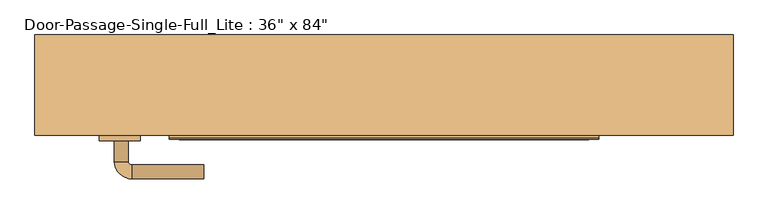
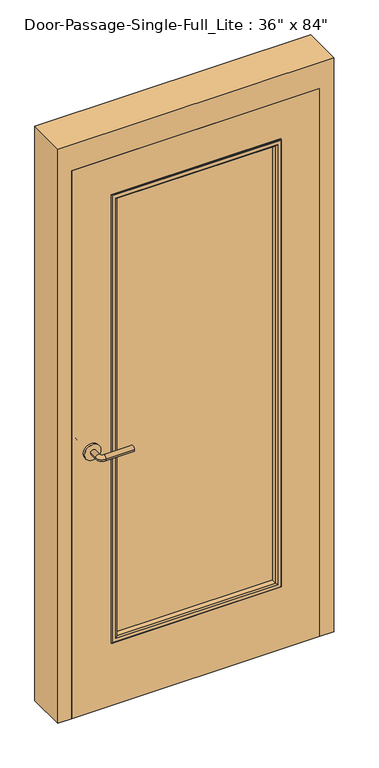
"""IFC4 building model written with IfcOpenShell, lengths in millimetres: door geometry."""

from ifc_helpers import new_model, si_unit, point, frame, frame_2d, origin, place, context, project, spatial, polyline, circle_curve, ellipse_curve, trimmed, segment, composite_curve, outline, extrude, faceted_brep, source, transform, mapped, element, save
from ifc_brep_helpers import plane_surface, cylinder_surface, revolved_surface, advanced_brep


def door_4cfbdd5f(model_context):
    return source(origin(), model_context, "Body", "SolidModel", [
        advanced_brep(
        [(-392.190625, -23.75, 1016.0), (-372.190625, -23.75, 1016.0), (-392.190625, 6.25, 1016.0), (-372.190625, 6.25, 1016.0), (-367.190625, 11.25, 1016.0), (-367.190625, 31.25, 1016.0), (-262.190625, 31.25, 1016.0), (-262.190625, 11.25, 1016.0)],
        [
            (0, 1, circle_curve(frame((-382.190625, -23.75, 1016.0), z_axis=(0.0, -1.0, 0.0), x_axis=(1.0, 0.0, 0.0)), 10.0)),
            (1, 0, circle_curve(frame((-382.190625, -23.75, 1016.0), z_axis=(0.0, -1.0, 0.0), x_axis=(1.0, 0.0, 0.0)), 10.0)),
            (0, 2),
            (2, 3, circle_curve(frame((-382.190625, 6.25, 1016.0), z_axis=(0.0, -1.0, 0.0), x_axis=(1.0, 0.0, 0.0)), 10.0)),
            (3, 1),
            (3, 2, circle_curve(frame((-382.190625, 6.25, 1016.0), z_axis=(0.0, -1.0, 0.0), x_axis=(1.0, 0.0, 0.0)), 10.0)),
            (4, 3, circle_curve(frame((-367.190625, 6.25, 1016.0), z_axis=(0.0, 0.0, 1.0), x_axis=(-1.0, 0.0, 0.0)), 5.0)),
            (2, 5, circle_curve(frame((-367.190625, 6.25, 1016.0), z_axis=(0.0, 0.0, -1.0), x_axis=(-1.0, 0.0, 0.0)), 25.0)),
            (5, 4, circle_curve(frame((-367.190625, 21.25, 1016.0), z_axis=(-1.0, 0.0, 0.0), x_axis=(0.0, -1.0, 0.0)), 10.0)),
            (4, 5, circle_curve(frame((-367.190625, 21.25, 1016.0), z_axis=(-1.0, 0.0, 0.0), x_axis=(0.0, -1.0, 0.0)), 10.0)),
            (6, 7, circle_curve(frame((-262.190625, 21.25, 1016.0), z_axis=(1.0, 0.0, 0.0), x_axis=(0.0, -1.0, 0.0)), 10.0)),
            (7, 6, circle_curve(frame((-262.190625, 21.25, 1016.0), z_axis=(1.0, 0.0, 0.0), x_axis=(0.0, -1.0, 0.0)), 10.0)),
            (5, 6),
            (7, 4),
        ],
        [
            plane_surface(frame((-382.190625, -23.75, 1016.0), z_axis=(0.0, -1.0, 0.0), x_axis=(0.0, 0.0, 1.0))),
            cylinder_surface(frame((-382.190625, -23.75, 1016.0), z_axis=(0.0, -1.0, 0.0), x_axis=(1.0, 0.0, 0.0)), 10.0),
            revolved_surface(trimmed(ellipse_curve(frame((-382.190625, 6.25, 1016.0), z_axis=(0.0, -1.0, 0.0), x_axis=(1.0, 0.0, 0.0)), 10.0, 10.0), [point((-392.190625, 6.25, 1016.0))], [point((-372.190625, 6.25, 1016.0))], True, "CARTESIAN"), (-367.190625, 6.25, 1016.0), (0.0, 0.0, -1.0)),
            revolved_surface(trimmed(ellipse_curve(frame((-382.190625, 6.25, 1016.0), z_axis=(0.0, -1.0, 0.0), x_axis=(1.0, 0.0, 0.0)), 10.0, 10.0), [point((-372.190625, 6.25, 1016.0))], [point((-392.190625, 6.25, 1016.0))], True, "CARTESIAN"), (-367.190625, 6.25, 1016.0), (0.0, 0.0, -1.0)),
            plane_surface(frame((-262.190625, 21.25, 1016.0), z_axis=(1.0, 0.0, 0.0), x_axis=(0.0, 0.0, 1.0))),
            cylinder_surface(frame((-367.190625, 21.25, 1016.0), z_axis=(-1.0, 0.0, 0.0), x_axis=(0.0, -1.0, 0.0)), 10.0),
        ],
        [
            (0, [[1, 2]]),
            (1, [[-1, 3, 4, 5]]),
            (1, [[-2, -5, 6, -3]]),
            (2, [[7, -4, 8, 9]]),
            (3, [[-8, -6, -7, 10]]),
            (4, [[11, 12]]),
            (5, [[-9, 13, -12, 14]]),
            (5, [[-10, -14, -11, -13]]),
        ],
    ),
        extrude(outline(composite_curve([segment(trimmed(circle_curve(frame_2d((1016.0, -384.690625)), 30.0), [point((1016.0, -414.690625))], [point((1016.0, -354.690625))], False, "CARTESIAN"), True, "CONTINUOUS"), segment(trimmed(circle_curve(frame_2d((1016.0, -384.690625)), 30.0), [point((1016.0, -354.690625))], [point((1016.0, -414.690625))], False, "CARTESIAN"), True, "CONTINUOUS")], self_intersect=False)), frame((0.0, -31.75, 0.0), z_axis=(0.0, 1.0, 0.0), x_axis=(0.0, 0.0, 1.0)), (0.0, 0.0, 1.0), 8.0),
        advanced_brep(
        [(-392.190625, -84.2, 1016.0), (-372.190625, -84.2, 1016.0), (-372.190625, -114.2, 1016.0), (-392.190625, -114.2, 1016.0), (-367.190625, -119.2, 1016.0), (-367.190625, -139.2, 1016.0), (-262.190625, -139.2, 1016.0), (-262.190625, -119.2, 1016.0)],
        [
            (0, 1, circle_curve(frame((-382.190625, -84.2, 1016.0), z_axis=(0.0, 1.0, 0.0), x_axis=(1.0, 0.0, 0.0)), 10.0)),
            (1, 0, circle_curve(frame((-382.190625, -84.2, 1016.0), z_axis=(0.0, 1.0, 0.0), x_axis=(1.0, 0.0, 0.0)), 10.0)),
            (1, 2),
            (2, 3, circle_curve(frame((-382.190625, -114.2, 1016.0), z_axis=(0.0, 1.0, 0.0), x_axis=(1.0, 0.0, 0.0)), 10.0)),
            (3, 0),
            (3, 2, circle_curve(frame((-382.190625, -114.2, 1016.0), z_axis=(0.0, 1.0, 0.0), x_axis=(1.0, 0.0, 0.0)), 10.0)),
            (4, 5, circle_curve(frame((-367.190625, -129.2, 1016.0), z_axis=(-1.0, 0.0, 0.0), x_axis=(0.0, 1.0, 0.0)), 10.0)),
            (5, 3, circle_curve(frame((-367.190625, -114.2, 1016.0), z_axis=(0.0, 0.0, -1.0), x_axis=(-1.0, 0.0, 0.0)), 25.0)),
            (2, 4, circle_curve(frame((-367.190625, -114.2, 1016.0), z_axis=(0.0, 0.0, 1.0), x_axis=(-1.0, 0.0, 0.0)), 5.0)),
            (5, 4, circle_curve(frame((-367.190625, -129.2, 1016.0), z_axis=(-1.0, 0.0, 0.0), x_axis=(0.0, 1.0, 0.0)), 10.0)),
            (6, 7, circle_curve(frame((-262.190625, -129.2, 1016.0), z_axis=(1.0, 0.0, 0.0), x_axis=(0.0, 1.0, 0.0)), 10.0)),
            (7, 6, circle_curve(frame((-262.190625, -129.2, 1016.0), z_axis=(1.0, 0.0, 0.0), x_axis=(0.0, 1.0, 0.0)), 10.0)),
            (4, 7),
            (6, 5),
        ],
        [
            plane_surface(frame((-382.190625, -84.2, 1016.0), z_axis=(0.0, 1.0, 0.0), x_axis=(0.0, 0.0, 1.0))),
            cylinder_surface(frame((-382.190625, -84.2, 1016.0), z_axis=(0.0, 1.0, 0.0), x_axis=(1.0, 0.0, 0.0)), 10.0),
            revolved_surface(trimmed(ellipse_curve(frame((-382.190625, -114.2, 1016.0), z_axis=(0.0, -1.0, 0.0), x_axis=(1.0, 0.0, 0.0)), 10.0, 10.0), [point((-392.190625, -114.2, 1016.0))], [point((-372.190625, -114.2, 1016.0))], True, "CARTESIAN"), (-367.190625, -114.2, 1016.0), (0.0, 0.0, -1.0)),
            revolved_surface(trimmed(ellipse_curve(frame((-382.190625, -114.2, 1016.0), z_axis=(0.0, -1.0, 0.0), x_axis=(1.0, 0.0, 0.0)), 10.0, 10.0), [point((-372.190625, -114.2, 1016.0))], [point((-392.190625, -114.2, 1016.0))], True, "CARTESIAN"), (-367.190625, -114.2, 1016.0), (0.0, 0.0, -1.0)),
            plane_surface(frame((-262.190625, -129.2, 1016.0), z_axis=(1.0, 0.0, 0.0), x_axis=(0.0, 0.0, 1.0))),
            cylinder_surface(frame((-367.190625, -129.2, 1016.0), z_axis=(-1.0, 0.0, 0.0), x_axis=(0.0, 1.0, 0.0)), 10.0),
        ],
        [
            (0, [[1, 2]]),
            (1, [[3, 4, 5, -2]]),
            (1, [[-5, 6, -3, -1]]),
            (2, [[7, 8, -4, 9]]),
            (3, [[10, -9, -6, -8]]),
            (4, [[11, 12]]),
            (5, [[13, -11, 14, -7]]),
            (5, [[-14, -12, -13, -10]]),
        ],
    ),
        extrude(outline(composite_curve([segment(trimmed(circle_curve(frame_2d((1016.0, -384.690625)), 30.0), [point((1016.0, -414.690625))], [point((1016.0, -354.690625))], False, "CARTESIAN"), True, "CONTINUOUS"), segment(trimmed(circle_curve(frame_2d((1016.0, -384.690625)), 30.0), [point((1016.0, -354.690625))], [point((1016.0, -414.690625))], False, "CARTESIAN"), True, "CONTINUOUS")], self_intersect=False)), frame((0.0, -84.2, 0.0), z_axis=(0.0, 1.0, 0.0), x_axis=(0.0, 0.0, 1.0)), (0.0, 0.0, 1.0), 8.0),
        extrude(outline(polyline([(304.8, -50.8), (304.8, -57.15), (-304.8, -57.15), (-304.8, -50.8), (304.8, -50.8)])), frame((0.0, 0.0, 254.0), z_axis=(0.0, 0.0, 1.0), x_axis=(1.0, 0.0, 0.0)), (0.0, 0.0, 1.0), 1727.2),
        faceted_brep([(457.2, -26.9875, 0.0), (441.325, -26.9875, 0.0), (441.325, 20.6375, 0.0), (457.2, 20.6375, 0.0), (457.2, 69.85, 0.0), (508.0, 69.85, 0.0), (508.0, -76.2, 0.0), (457.2, -76.2, 0.0), (457.2, -76.2, 2133.6), (457.2, -26.9875, 2133.6), (508.0, -76.2, 2235.2), (-508.0, -76.2, 2235.2), (-508.0, -76.2, 0.0), (-457.2, -76.2, 0.0), (-457.2, -76.2, 2133.6), (508.0, 69.85, 2235.2), (457.2, 69.85, 2133.6), (-457.2, 69.85, 2133.6), (-457.2, 69.85, 0.0), (-508.0, 69.85, 0.0), (-508.0, 69.85, 2235.2), (457.2, 20.6375, 2133.6), (441.325, 20.6375, 2117.725), (-441.325, 20.6375, 2117.725), (-441.325, 20.6375, 0.0), (-457.2, 20.6375, 0.0), (-457.2, 20.6375, 2133.6), (441.325, -26.9875, 2117.725), (-457.2, -26.9875, 2133.6), (-457.2, -26.9875, 0.0), (-441.325, -26.9875, 0.0), (-441.325, -26.9875, 2117.725)], [[[0, 1, 2, 3, 4, 5, 6, 7]], [[7, 8, 9, 0]], [[6, 10, 11, 12, 13, 14, 8, 7]], [[5, 15, 10, 6]], [[4, 16, 17, 18, 19, 20, 15, 5]], [[3, 21, 16, 4]], [[2, 22, 23, 24, 25, 26, 21, 3]], [[1, 27, 22, 2]], [[0, 9, 28, 29, 30, 31, 27, 1]], [[8, 14, 28, 9]], [[16, 21, 26, 17]], [[22, 27, 31, 23]], [[12, 19, 18, 25, 24, 30, 29, 13]], [[13, 29, 28, 14]], [[11, 20, 19, 12]], [[17, 26, 25, 18]], [[23, 31, 30, 24]], [[15, 20, 11, 10]]]),
        extrude(outline(polyline([(2133.6, -457.2), (0.0, -457.2), (0.0, 457.2), (2133.6, 457.2), (2133.6, -457.2)]), holes=[polyline([(1981.2, -304.8), (1981.2, 304.8), (254.0, 304.8), (254.0, -304.8), (1981.2, -304.8)])]), frame((0.0, -76.2, 0.0), z_axis=(0.0, 1.0, 0.0), x_axis=(0.0, 0.0, 1.0)), (0.0, 0.0, 1.0), 44.45),
        advanced_brep(
        [(-304.8, -57.15, 1981.2), (-304.8, -57.15, 254.0), (-304.8, -76.2, 254.0), (-304.8, -76.2, 1981.2), (-292.8, -77.2, 1969.2), (-292.8, -77.2, 266.0), (-292.8, -57.15, 266.0), (-292.8, -57.15, 1969.2), (-297.8, -82.2, 1974.2), (-297.8, -82.2, 261.0), (-312.8, -80.2, 1989.2), (-312.8, -80.2, 246.0), (-310.8, -82.2, 248.0), (-310.8, -82.2, 1987.2), (-312.8, -76.2, 1989.2), (-312.8, -76.2, 246.0), (304.8, -57.15, 254.0), (304.8, -76.2, 254.0), (292.8, -77.2, 266.0), (292.8, -57.15, 266.0), (297.8, -82.2, 261.0), (312.8, -80.2, 246.0), (310.8, -82.2, 248.0), (312.8, -76.2, 246.0), (304.8, -57.15, 1981.2), (304.8, -76.2, 1981.2), (292.8, -77.2, 1969.2), (292.8, -57.15, 1969.2), (297.8, -82.2, 1974.2), (312.8, -80.2, 1989.2), (310.8, -82.2, 1987.2), (312.8, -76.2, 1989.2)],
        [
            (0, 1),
            (1, 2),
            (2, 3),
            (3, 0),
            (4, 5),
            (5, 6),
            (6, 7),
            (7, 4),
            (8, 9),
            (9, 5, ellipse_curve(frame((-297.8, -77.2, 261.0), z_axis=(-0.7071067811865475, 0.0, 0.7071067811865475), x_axis=(0.7071067811865474, 0.0, 0.7071067811865476)), 7.0710678, 5.0)),
            (4, 8, ellipse_curve(frame((-297.8, -77.2, 1974.2), z_axis=(-0.7071067811865475, 0.0, -0.7071067811865475), x_axis=(-0.7071067811865474, 0.0, 0.7071067811865476)), 7.0710678, 5.0)),
            (10, 11),
            (11, 12, ellipse_curve(frame((-310.8, -80.2, 248.0), z_axis=(-0.7071067811865475, 0.0, 0.7071067811865475), x_axis=(0.7071067811865474, 0.0, 0.7071067811865476)), 2.8284271, 2.0)),
            (12, 13),
            (13, 10, ellipse_curve(frame((-310.8, -80.2, 1987.2), z_axis=(-0.7071067811865475, 0.0, -0.7071067811865475), x_axis=(-0.7071067811865474, 0.0, 0.7071067811865476)), 2.8284271, 2.0)),
            (14, 15),
            (15, 11),
            (10, 14),
            (1, 16),
            (16, 17),
            (17, 2),
            (5, 18),
            (18, 19),
            (19, 6),
            (9, 20),
            (20, 18, ellipse_curve(frame((297.8, -77.2, 261.0), z_axis=(-0.7071067811865475, 0.0, -0.7071067811865475), x_axis=(-0.7071067811865476, 0.0, 0.7071067811865474)), 7.0710678, 5.0)),
            (11, 21),
            (21, 22, ellipse_curve(frame((310.8, -80.2, 248.0), z_axis=(-0.7071067811865475, 0.0, -0.7071067811865475), x_axis=(-0.7071067811865476, 0.0, 0.7071067811865474)), 2.8284271, 2.0)),
            (22, 12),
            (15, 23),
            (23, 21),
            (16, 24),
            (24, 25),
            (25, 17),
            (18, 26),
            (26, 27),
            (27, 19),
            (20, 28),
            (28, 26, ellipse_curve(frame((297.8, -77.2, 1974.2), z_axis=(0.7071067811865475, 0.0, -0.7071067811865475), x_axis=(-0.7071067811865474, 0.0, -0.7071067811865476)), 7.0710678, 5.0)),
            (21, 29),
            (29, 30, ellipse_curve(frame((310.8, -80.2, 1987.2), z_axis=(0.7071067811865475, 0.0, -0.7071067811865475), x_axis=(-0.7071067811865474, 0.0, -0.7071067811865476)), 2.8284271, 2.0)),
            (30, 22),
            (23, 31),
            (31, 29),
            (14, 31),
            (25, 3),
            (24, 0),
            (27, 7),
            (26, 4),
            (28, 8),
            (30, 13),
            (29, 10),
        ],
        [
            plane_surface(frame((-304.8, -76.2, 1981.2), z_axis=(-1.0, 0.0, 0.0), x_axis=(0.0, 0.0, -1.0))),
            plane_surface(frame((-292.8, -57.15, 1969.2), z_axis=(1.0, 0.0, 0.0), x_axis=(0.0, 0.0, -1.0))),
            cylinder_surface(frame((-297.8, -77.2, 1981.2), z_axis=(0.0, 0.0, 1.0), x_axis=(-1.0, 0.0, 0.0)), 5.0),
            cylinder_surface(frame((-310.8, -80.2, 1981.2), z_axis=(0.0, 0.0, 1.0), x_axis=(-1.0, 0.0, 0.0)), 2.0),
            plane_surface(frame((-312.8, -80.2, 1989.2), z_axis=(-1.0, 0.0, 0.0), x_axis=(0.0, 0.0, -1.0))),
            plane_surface(frame((-304.8, -76.2, 254.0), z_axis=(0.0, 0.0, -1.0), x_axis=(1.0, 0.0, 0.0))),
            plane_surface(frame((-292.8, -57.15, 266.0), z_axis=(0.0, 0.0, 1.0), x_axis=(1.0, 0.0, 0.0))),
            cylinder_surface(frame((-304.8, -77.2, 261.0), z_axis=(-1.0, 0.0, 0.0), x_axis=(0.0, 0.0, -1.0)), 5.0),
            cylinder_surface(frame((-304.8, -80.2, 248.0), z_axis=(-1.0, 0.0, 0.0), x_axis=(0.0, 0.0, -1.0)), 2.0),
            plane_surface(frame((-312.8, -80.2, 246.0), z_axis=(0.0, 0.0, -1.0), x_axis=(1.0, 0.0, 0.0))),
            plane_surface(frame((304.8, -76.2, 254.0), z_axis=(1.0, 0.0, 0.0), x_axis=(0.0, 0.0, 1.0))),
            plane_surface(frame((292.8, -57.15, 266.0), z_axis=(-1.0, 0.0, 0.0), x_axis=(0.0, 0.0, 1.0))),
            cylinder_surface(frame((297.8, -77.2, 254.0), z_axis=(0.0, 0.0, -1.0), x_axis=(1.0, 0.0, 0.0)), 5.0),
            cylinder_surface(frame((310.8, -80.2, 254.0), z_axis=(0.0, 0.0, -1.0), x_axis=(1.0, 0.0, 0.0)), 2.0),
            plane_surface(frame((312.8, -80.2, 246.0), z_axis=(1.0, 0.0, 0.0), x_axis=(0.0, 0.0, 1.0))),
            plane_surface(frame((312.8, -76.2, 1989.2), z_axis=(0.0, 1.0, 0.0), x_axis=(-1.0, 0.0, 0.0))),
            plane_surface(frame((304.8, -76.2, 1981.2), z_axis=(0.0, 0.0, 1.0), x_axis=(-1.0, 0.0, 0.0))),
            plane_surface(frame((304.8, -57.15, 1981.2), z_axis=(0.0, 1.0, 0.0), x_axis=(-1.0, 0.0, 0.0))),
            plane_surface(frame((292.8, -57.15, 1969.2), z_axis=(0.0, 0.0, -1.0), x_axis=(-1.0, 0.0, 0.0))),
            cylinder_surface(frame((304.8, -77.2, 1974.2), z_axis=(1.0, 0.0, 0.0), x_axis=(0.0, 0.0, 1.0)), 5.0),
            plane_surface(frame((297.8, -82.2, 1974.2), z_axis=(0.0, -1.0, 0.0), x_axis=(-1.0, 0.0, 0.0))),
            cylinder_surface(frame((304.8, -80.2, 1987.2), z_axis=(1.0, 0.0, 0.0), x_axis=(0.0, 0.0, 1.0)), 2.0),
            plane_surface(frame((312.8, -80.2, 1989.2), z_axis=(0.0, 0.0, 1.0), x_axis=(-1.0, 0.0, 0.0))),
        ],
        [
            (0, [[1, 2, 3, 4]]),
            (1, [[5, 6, 7, 8]]),
            (2, [[9, 10, -5, 11]]),
            (3, [[12, 13, 14, 15]]),
            (4, [[16, 17, -12, 18]]),
            (5, [[19, 20, 21, -2]]),
            (6, [[22, 23, 24, -6]]),
            (7, [[25, 26, -22, -10]]),
            (8, [[27, 28, 29, -13]]),
            (9, [[30, 31, -27, -17]]),
            (10, [[32, 33, 34, -20]]),
            (11, [[35, 36, 37, -23]]),
            (12, [[38, 39, -35, -26]]),
            (13, [[40, 41, 42, -28]]),
            (14, [[43, 44, -40, -31]]),
            (15, [[-16, 45, -43, -30], [-3, -21, -34, 46]]),
            (16, [[47, -4, -46, -33]]),
            (17, [[-1, -47, -32, -19], [-7, -24, -37, 48]]),
            (18, [[49, -8, -48, -36]]),
            (19, [[50, -11, -49, -39]]),
            (20, [[-14, -29, -42, 51], [-9, -50, -38, -25]]),
            (21, [[52, -15, -51, -41]]),
            (22, [[-45, -18, -52, -44]]),
        ],
    ),
        advanced_brep(
        [(-304.8, -50.8, 254.0), (-304.8, -50.8, 1981.2), (-304.8, -31.75, 1981.2), (-304.8, -31.75, 254.0), (-292.8, -30.75, 266.0), (-292.8, -30.75, 1969.2), (-292.8, -50.8, 1969.2), (-292.8, -50.8, 266.0), (-297.8, -25.75, 261.0), (-297.8, -25.75, 1974.2), (-312.8, -27.75, 246.0), (-312.8, -27.75, 1989.2), (-310.8, -25.75, 1987.2), (-310.8, -25.75, 248.0), (-312.8, -31.75, 246.0), (-312.8, -31.75, 1989.2), (304.8, -50.8, 1981.2), (304.8, -31.75, 1981.2), (292.8, -30.75, 1969.2), (292.8, -50.8, 1969.2), (297.8, -25.75, 1974.2), (312.8, -27.75, 1989.2), (310.8, -25.75, 1987.2), (312.8, -31.75, 1989.2), (304.8, -50.8, 254.0), (304.8, -31.75, 254.0), (292.8, -30.75, 266.0), (292.8, -50.8, 266.0), (297.8, -25.75, 261.0), (312.8, -27.75, 246.0), (310.8, -25.75, 248.0), (312.8, -31.75, 246.0)],
        [
            (0, 1),
            (1, 2),
            (2, 3),
            (3, 0),
            (4, 5),
            (5, 6),
            (6, 7),
            (7, 4),
            (8, 9),
            (9, 5, ellipse_curve(frame((-297.8, -30.75, 1974.2), z_axis=(-0.7071067811865475, 0.0, -0.7071067811865475), x_axis=(0.7071067811865474, 0.0, -0.7071067811865476)), 7.0710678, 5.0)),
            (4, 8, ellipse_curve(frame((-297.8, -30.75, 261.0), z_axis=(-0.7071067811865475, 0.0, 0.7071067811865475), x_axis=(-0.7071067811865474, 0.0, -0.7071067811865476)), 7.0710678, 5.0)),
            (10, 11),
            (11, 12, ellipse_curve(frame((-310.8, -27.75, 1987.2), z_axis=(-0.7071067811865475, 0.0, -0.7071067811865475), x_axis=(0.7071067811865474, 0.0, -0.7071067811865476)), 2.8284271, 2.0)),
            (12, 13),
            (13, 10, ellipse_curve(frame((-310.8, -27.75, 248.0), z_axis=(-0.7071067811865475, 0.0, 0.7071067811865475), x_axis=(-0.7071067811865474, 0.0, -0.7071067811865476)), 2.8284271, 2.0)),
            (14, 15),
            (15, 11),
            (10, 14),
            (1, 16),
            (16, 17),
            (17, 2),
            (5, 18),
            (18, 19),
            (19, 6),
            (9, 20),
            (20, 18, ellipse_curve(frame((297.8, -30.75, 1974.2), z_axis=(-0.7071067811865475, 0.0, 0.7071067811865475), x_axis=(-0.7071067811865476, 0.0, -0.7071067811865474)), 7.0710678, 5.0)),
            (11, 21),
            (21, 22, ellipse_curve(frame((310.8, -27.75, 1987.2), z_axis=(-0.7071067811865475, 0.0, 0.7071067811865475), x_axis=(-0.7071067811865476, 0.0, -0.7071067811865474)), 2.8284271, 2.0)),
            (22, 12),
            (15, 23),
            (23, 21),
            (16, 24),
            (24, 25),
            (25, 17),
            (18, 26),
            (26, 27),
            (27, 19),
            (20, 28),
            (28, 26, ellipse_curve(frame((297.8, -30.75, 261.0), z_axis=(0.7071067811865475, 0.0, 0.7071067811865475), x_axis=(-0.7071067811865474, 0.0, 0.7071067811865476)), 7.0710678, 5.0)),
            (21, 29),
            (29, 30, ellipse_curve(frame((310.8, -27.75, 248.0), z_axis=(0.7071067811865475, 0.0, 0.7071067811865475), x_axis=(-0.7071067811865474, 0.0, 0.7071067811865476)), 2.8284271, 2.0)),
            (30, 22),
            (23, 31),
            (31, 29),
            (14, 31),
            (25, 3),
            (24, 0),
            (27, 7),
            (26, 4),
            (28, 8),
            (30, 13),
            (29, 10),
        ],
        [
            plane_surface(frame((-304.8, -31.75, 254.0), z_axis=(-1.0, 0.0, 0.0), x_axis=(0.0, 0.0, 1.0))),
            plane_surface(frame((-292.8, -50.8, 266.0), z_axis=(1.0, 0.0, 0.0), x_axis=(0.0, 0.0, 1.0))),
            cylinder_surface(frame((-297.8, -30.75, 254.0), z_axis=(0.0, 0.0, -1.0), x_axis=(-1.0, 0.0, 0.0)), 5.0),
            cylinder_surface(frame((-310.8, -27.75, 254.0), z_axis=(0.0, 0.0, -1.0), x_axis=(-1.0, 0.0, 0.0)), 2.0),
            plane_surface(frame((-312.8, -27.75, 246.0), z_axis=(-1.0, 0.0, 0.0), x_axis=(0.0, 0.0, 1.0))),
            plane_surface(frame((-304.8, -31.75, 1981.2), z_axis=(0.0, 0.0, 1.0), x_axis=(1.0, 0.0, 0.0))),
            plane_surface(frame((-292.8, -50.8, 1969.2), z_axis=(0.0, 0.0, -1.0), x_axis=(1.0, 0.0, 0.0))),
            cylinder_surface(frame((-304.8, -30.75, 1974.2), z_axis=(-1.0, 0.0, 0.0), x_axis=(0.0, 0.0, 1.0)), 5.0),
            cylinder_surface(frame((-304.8, -27.75, 1987.2), z_axis=(-1.0, 0.0, 0.0), x_axis=(0.0, 0.0, 1.0)), 2.0),
            plane_surface(frame((-312.8, -27.75, 1989.2), z_axis=(0.0, 0.0, 1.0), x_axis=(1.0, 0.0, 0.0))),
            plane_surface(frame((304.8, -31.75, 1981.2), z_axis=(1.0, 0.0, 0.0), x_axis=(0.0, 0.0, -1.0))),
            plane_surface(frame((292.8, -50.8, 1969.2), z_axis=(-1.0, 0.0, 0.0), x_axis=(0.0, 0.0, -1.0))),
            cylinder_surface(frame((297.8, -30.75, 1981.2), z_axis=(0.0, 0.0, 1.0), x_axis=(1.0, 0.0, 0.0)), 5.0),
            cylinder_surface(frame((310.8, -27.75, 1981.2), z_axis=(0.0, 0.0, 1.0), x_axis=(1.0, 0.0, 0.0)), 2.0),
            plane_surface(frame((312.8, -27.75, 1989.2), z_axis=(1.0, 0.0, 0.0), x_axis=(0.0, 0.0, -1.0))),
            plane_surface(frame((312.8, -31.75, 246.0), z_axis=(0.0, -1.0, 0.0), x_axis=(-1.0, 0.0, 0.0))),
            plane_surface(frame((304.8, -31.75, 254.0), z_axis=(0.0, 0.0, -1.0), x_axis=(-1.0, 0.0, 0.0))),
            plane_surface(frame((304.8, -50.8, 254.0), z_axis=(0.0, -1.0, 0.0), x_axis=(-1.0, 0.0, 0.0))),
            plane_surface(frame((292.8, -50.8, 266.0), z_axis=(0.0, 0.0, 1.0), x_axis=(-1.0, 0.0, 0.0))),
            cylinder_surface(frame((304.8, -30.75, 261.0), z_axis=(1.0, 0.0, 0.0), x_axis=(0.0, 0.0, -1.0)), 5.0),
            plane_surface(frame((297.8, -25.75, 261.0), z_axis=(0.0, 1.0, 0.0), x_axis=(-1.0, 0.0, 0.0))),
            cylinder_surface(frame((304.8, -27.75, 248.0), z_axis=(1.0, 0.0, 0.0), x_axis=(0.0, 0.0, -1.0)), 2.0),
            plane_surface(frame((312.8, -27.75, 246.0), z_axis=(0.0, 0.0, -1.0), x_axis=(-1.0, 0.0, 0.0))),
        ],
        [
            (0, [[1, 2, 3, 4]]),
            (1, [[5, 6, 7, 8]]),
            (2, [[9, 10, -5, 11]]),
            (3, [[12, 13, 14, 15]]),
            (4, [[16, 17, -12, 18]]),
            (5, [[19, 20, 21, -2]]),
            (6, [[22, 23, 24, -6]]),
            (7, [[25, 26, -22, -10]]),
            (8, [[27, 28, 29, -13]]),
            (9, [[30, 31, -27, -17]]),
            (10, [[32, 33, 34, -20]]),
            (11, [[35, 36, 37, -23]]),
            (12, [[38, 39, -35, -26]]),
            (13, [[40, 41, 42, -28]]),
            (14, [[43, 44, -40, -31]]),
            (15, [[-16, 45, -43, -30], [-3, -21, -34, 46]]),
            (16, [[47, -4, -46, -33]]),
            (17, [[-1, -47, -32, -19], [-7, -24, -37, 48]]),
            (18, [[49, -8, -48, -36]]),
            (19, [[50, -11, -49, -39]]),
            (20, [[-14, -29, -42, 51], [-9, -50, -38, -25]]),
            (21, [[52, -15, -51, -41]]),
            (22, [[-45, -18, -52, -44]]),
        ],
    ),
    ])


if __name__ == "__main__":
    model = new_model("IFC4")
    model_context = context("Model", 3, world=origin())
    ifc_project = project(units=[si_unit("LENGTHUNIT", "METRE", prefix="MILLI")], contexts=[model_context])
    site = spatial("IfcSite", under=ifc_project)
    building = spatial("IfcBuilding", under=site)
    placement = place(None, origin())
    door_shape = door_4cfbdd5f(model_context)
    element("IfcDoor", 1, ObjectType="Door-Passage-Single-Full_Lite : 36\" x 84\"", at=placement, inside=building, context=model_context, shape_type="MappedRepresentation", body=[
        mapped(door_shape, transform((0.0, 0.0, 0.0), x_axis=(1.0, 0.0, 0.0), y_axis=(0.0, 1.0, 0.0), z_axis=(0.0, 0.0, 1.0))),
    ])
    save(model, "model.ifc")

# Revit data of these elements
# Type "Door-Passage-Single-Full_Lite : 36\" x 84\""
#   Type Mark = "52"
#   Assembly Code = "B2030100"
#   Analytic Construction = "Wooden"
#   Thickness = 0' - 1 3/4"
#   Thermal Resistance (R) = 2.5876 (h·ft²·°F)/BTU
#   Swing Angle [instance default] = 90.00°
#   Strike Height = 3' - 4"
#   Rough Width [instance default] = 3' - 4"
#   Rough Height [instance default] = 7' - 4"
#   MF Opening Height [instance default] = 0' - 4"
#   MF Opening Width [instance default] = 0' - 4"
#   Inset Calculate [instance default] = 0' - 4"
#   Masonry Inset [instance default] = 0' - 1"
#   Height = 7' - 0"
#   Width = 3' - 0"
#   Heat Transfer Coefficient (U) = 0.3865 BTU/(h·ft²·°F)
#   Masonry Frame Depth = 0' - 5 3/4"
#   Masonry Frame [instance default] = yes
#   Function = 1
#   Dry Wall Frame [instance default] = no
#   Panel Material = Wood - Birch
#   Glazing = Glass
#   Glass Stop Material = Metal - Paint Finish - Grey
#   Frame Material = Metal - Paint Finish - Grey
#   Door Handle Material = Aluminum
#   Visual Light Transmittance = 0
#   Solar Heat Gain Coefficient = 0
#   Wall Closure = (empty or 0)
# Element 1 (IfcDoor, "Door-Passage-Single-Full_Lite : 36\" x 84\"")
#   Inset Calculate = 0' - 3"
#   Masonry Inset = 0' - 0"
#   Materials on its faces: "Metal - Paint Finish - Grey", "Aluminum", "Wood - Birch", "Glass"
# Materials
#   "Wood - Birch": class "Wood", colour RGB 166 116 52, transparency 0, Cost = 0
#   "Glass": class "Glass", colour RGB 0 128 192, transparency 0.75, Description = "Soda Lime Glass", Cost = 0
#   "Metal - Paint Finish - Grey": class "Paint", colour RGB 104 104 104, transparency 0, Cost = 0
#   "Aluminum": class "Metal", colour RGB 247 247 247, transparency 0, Description = "Aluminum 6061", Cost = 0
